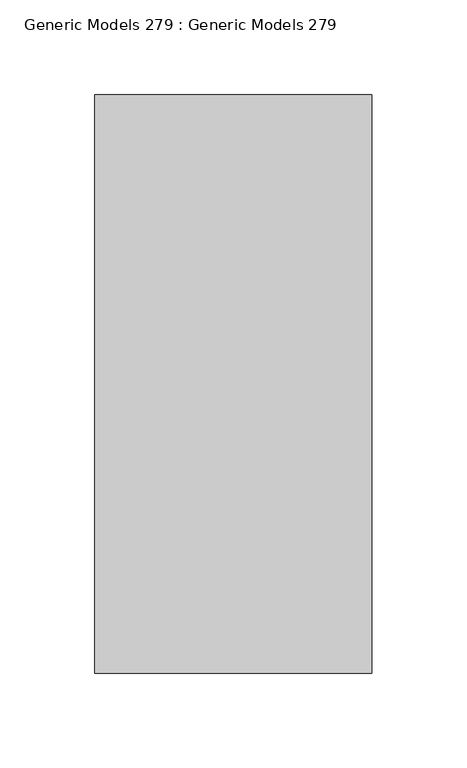
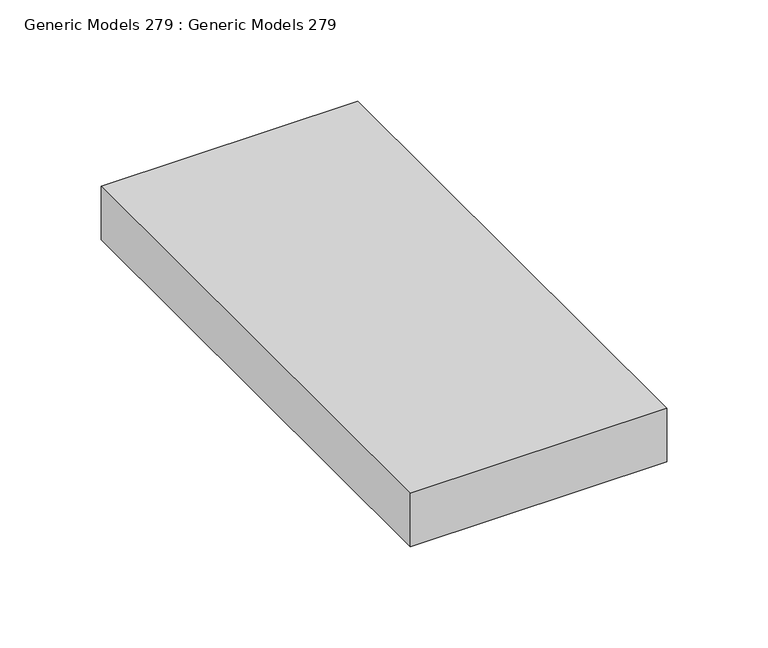
"""IFC4 building model written with IfcOpenShell, lengths in millimetres: proxy geometry, Generic Models 279 : Generic Models 279."""

import ifcopenshell
import ifcopenshell.guid

model = None  # the IFC model being written
_history = None  # IfcOwnerHistory: only IFC2X3 demands one
_inside = {}  # id of a spatial element -> (the spatial element, [elements in it])
_under = {}  # id of a project, library or spatial element -> (it, [spatial elements below it])
_declared = {}  # id of a project -> (the project, [libraries it declares])
_typed = {}  # id of a type object -> (the type object, [elements of that type])
_made_of = {}  # id of a material, layer set ... -> (it, [elements and type objects made of it])


def new_model(schema):
    """Start an empty IFC model of exactly this schema.

    Asked for "IFC4X3", IfcOpenShell would pick the latest addendum, in which some entities
    have other attributes; the version numbers below select the first issue.
    IFC2X3 requires an IfcOwnerHistory on every rooted entity: one is made here for all.
    """
    global model, _history
    if schema == "IFC4X3":
        model = ifcopenshell.file(schema_version=(4, 3, 0, 0))
    else:
        model = ifcopenshell.file(schema=schema)
    _inside.clear()
    _under.clear()
    _declared.clear()
    _typed.clear()
    _made_of.clear()
    _history = None
    if model.schema == "IFC2X3":
        org = make("IfcOrganization", Name="unknown")
        user = make(
            "IfcPersonAndOrganization",
            ThePerson=make("IfcPerson", FamilyName="unknown"),
            TheOrganization=org,
        )
        app = make(
            "IfcApplication",
            ApplicationDeveloper=org,
            Version="unknown",
            ApplicationFullName="unknown",
            ApplicationIdentifier="unknown",
        )
        _history = make(
            "IfcOwnerHistory",
            OwningUser=user,
            OwningApplication=app,
            ChangeAction="ADDED",
            CreationDate=0,
        )
    return model


def make(cls, **values):
    """One entity of the class cls with the attributes given. An attribute that is None is left unset."""
    return model.create_entity(
        cls, **{name: value for name, value in values.items() if value is not None}
    )


def rooted(cls, **values):
    """An entity with a GlobalId (a new one), such as an element, a storey or a relation."""
    return make(cls, GlobalId=ifcopenshell.guid.new(), OwnerHistory=_history, **values)


def si_unit(unit_type, name, prefix=None):
    """IfcSIUnit, for example si_unit("LENGTHUNIT", "METRE", prefix="MILLI")."""
    return make("IfcSIUnit", UnitType=unit_type, Prefix=prefix, Name=name)


def assignment(units):
    """IfcUnitAssignment: the units of a project."""
    return None if units is None else make("IfcUnitAssignment", Units=units)


def point(xyz):
    """IfcCartesianPoint."""
    return None if xyz is None else make("IfcCartesianPoint", Coordinates=xyz)


def direction(xyz):
    """IfcDirection."""
    return None if xyz is None else make("IfcDirection", DirectionRatios=xyz)


def frame(location, z_axis=None, x_axis=None):
    """IfcAxis2Placement3D, a coordinate frame: its origin and axes. An axis left out is left unset."""
    return make(
        "IfcAxis2Placement3D",
        Location=point(location),
        Axis=direction(z_axis),
        RefDirection=direction(x_axis),
    )


def origin():
    """The frame at (0, 0, 0) with its axes left unset."""
    return frame((0.0, 0.0, 0.0))


def place(relative_to, where):
    """IfcLocalPlacement: puts the frame where relative to a parent placement (None: the world)."""
    return make(
        "IfcLocalPlacement", PlacementRelTo=relative_to, RelativePlacement=where
    )


def context(
    kind, dimensions, precision=None, world=None, true_north=None, identifier=None
):
    """IfcGeometricRepresentationContext, for example the 3D "Model" context."""
    return make(
        "IfcGeometricRepresentationContext",
        ContextIdentifier=identifier,
        ContextType=kind,
        CoordinateSpaceDimension=dimensions,
        Precision=precision,
        WorldCoordinateSystem=world,
        TrueNorth=true_north,
    )


def project(units=None, contexts=None):
    """IfcProject with its units and contexts."""
    return rooted(
        "IfcProject",
        Name="project",
        RepresentationContexts=contexts,
        UnitsInContext=assignment(units),
    )


def spatial(cls, under=None, at=None, **own):
    """A site, building, storey or space (cls), placed at a placement, below another one or the project."""
    s = rooted(cls, ObjectPlacement=at, **own)
    if under is not None:
        _under.setdefault(under.id(), (under, []))[1].append(s)
    return s


def polyline(points):
    """IfcPolyline through the points."""
    return make("IfcPolyline", Points=[point(p) for p in points])


def outline(outer, holes=None, kind="AREA"):
    """IfcArbitraryClosedProfileDef: a profile drawn as a closed curve; with holes, ...WithVoids."""
    if holes is None:
        return make("IfcArbitraryClosedProfileDef", ProfileType=kind, OuterCurve=outer)
    return make(
        "IfcArbitraryProfileDefWithVoids",
        ProfileType=kind,
        OuterCurve=outer,
        InnerCurves=holes,
    )


def extrude(swept, where, along, depth):
    """IfcExtrudedAreaSolid: the profile swept, set in the frame where, extruded along a direction by depth."""
    return make(
        "IfcExtrudedAreaSolid",
        SweptArea=swept,
        Position=where,
        ExtrudedDirection=direction(along),
        Depth=depth,
    )


def shape(context_of_items, identifier, shape_type, items):
    """IfcShapeRepresentation: the items that make up one representation, for example the "Body"."""
    return make(
        "IfcShapeRepresentation",
        ContextOfItems=context_of_items,
        RepresentationIdentifier=identifier,
        RepresentationType=shape_type,
        Items=items,
    )


def source(mapping_origin, context_of_items, identifier, shape_type, items):
    """IfcRepresentationMap: a shape defined once, which mapped items show again and again."""
    return make(
        "IfcRepresentationMap",
        MappingOrigin=mapping_origin,
        MappedRepresentation=shape(context_of_items, identifier, shape_type, items),
    )


def transform(
    local_origin,
    x_axis=None,
    y_axis=None,
    z_axis=None,
    scale=None,
    scale2=None,
    scale3=None,
    uniform=True,
):
    """IfcCartesianTransformationOperator3D, or its non-uniform kind. x_axis, y_axis, z_axis: its Axis1, 2, 3."""
    if uniform:
        return make(
            "IfcCartesianTransformationOperator3D",
            Axis1=direction(x_axis),
            Axis2=direction(y_axis),
            LocalOrigin=point(local_origin),
            Scale=scale,
            Axis3=direction(z_axis),
        )
    return make(
        "IfcCartesianTransformationOperator3DnonUniform",
        Axis1=direction(x_axis),
        Axis2=direction(y_axis),
        LocalOrigin=point(local_origin),
        Scale=scale,
        Axis3=direction(z_axis),
        Scale2=scale2,
        Scale3=scale3,
    )


def mapped(mapping_source, mapping_target):
    """IfcMappedItem: shows the shape of a source again, moved by a transform."""
    return make(
        "IfcMappedItem", MappingSource=mapping_source, MappingTarget=mapping_target
    )


def made_of(thing, what):
    """Note that an element or type object is made of a material, layer set ...; save() writes the relation."""
    if what is not None:
        _made_of.setdefault(what.id(), (what, []))[1].append(thing)
    return thing


def element(
    cls,
    number,
    at=None,
    inside=None,
    cuts=None,
    type_object=None,
    material=None,
    context=None,
    identifier="Body",
    shape_type=None,
    held_by="IfcProductDefinitionShape",
    body=None,
    shapes=None,
    **own,
):
    """One element of the class cls, such as IfcWall. Its Tag is "e" and its number.

    at: its placement. inside: the storey or other place that contains it. cuts: it is an
    opening in that element (IfcRelVoidsElement). A single representation is given by context,
    identifier, shape_type and body (its items); several are given by shapes. held_by: the class
    of the entity that holds the representations. save() writes the other relations.
    """
    e = rooted(cls, Tag="e%d" % number, ObjectPlacement=at, **own)
    if body is not None:
        shapes = [shape(context, identifier, shape_type, body)]
    if shapes is not None:
        e.Representation = make(held_by, Representations=shapes)
    if inside is not None:
        _inside.setdefault(inside.id(), (inside, []))[1].append(e)
    if cuts is not None:
        rooted(
            "IfcRelVoidsElement", RelatingBuildingElement=cuts, RelatedOpeningElement=e
        )
    if type_object is not None:
        _typed.setdefault(type_object.id(), (type_object, []))[1].append(e)
    return made_of(e, material)


def aggregate(whole, parts):
    """IfcRelAggregates: a whole, such as a stair, and the parts it consists of."""
    return rooted("IfcRelAggregates", RelatingObject=whole, RelatedObjects=parts)


def save(model, path):
    """Write the relations noted so far, then the file.

    IfcRelAggregates (storeys below a building ...), IfcRelContainedInSpatialStructure (elements
    in a storey), IfcRelDefinesByType, IfcRelAssociatesMaterial and IfcRelDeclares: one each for
    every whole, place, type object, material and project.
    """
    for whole, parts in _under.values():
        aggregate(whole, parts)
    for where, things in _inside.values():
        rooted(
            "IfcRelContainedInSpatialStructure",
            RelatedElements=things,
            RelatingStructure=where,
        )
    for kind, things in _typed.values():
        rooted("IfcRelDefinesByType", RelatedObjects=things, RelatingType=kind)
    for what, things in _made_of.values():
        rooted("IfcRelAssociatesMaterial", RelatedObjects=things, RelatingMaterial=what)
    for by, libraries in _declared.values():
        rooted("IfcRelDeclares", RelatingContext=by, RelatedDefinitions=libraries)
    model.write(path)


def generic_models_279_generic_models_279_9df74be8(model_context):
    return source(origin(), model_context, "Body", "SweptSolid", [
        extrude(outline(polyline([(3531.1804357, 704.5309662), (3677.2304357, 704.5309662), (3677.2304357, 399.7309662), (3531.1804357, 399.7309662), (3531.1804357, 704.5309662)])), frame((0.0, 0.0, 124745.2775398), z_axis=(0.0, 0.0, 1.0), x_axis=(1.0, 0.0, 0.0)), (0.0, 0.0, 1.0), 32.1869688),
    ])


if __name__ == "__main__":
    model = new_model("IFC4")
    model_context = context("Model", 3, world=origin())
    ifc_project = project(units=[si_unit("LENGTHUNIT", "METRE", prefix="MILLI")], contexts=[model_context])
    site = spatial("IfcSite", under=ifc_project)
    building = spatial("IfcBuilding", under=site)
    placement = place(None, origin())
    generic_models_279_generic_models_279_shape = generic_models_279_generic_models_279_9df74be8(model_context)
    element("IfcBuildingElementProxy", 1, Name="Generic Models 279 : Generic Models 279", ObjectType="Generic Models 279 : Generic Models 279", at=placement, inside=building, context=model_context, shape_type="MappedRepresentation", body=[
        mapped(generic_models_279_generic_models_279_shape, transform((0.0, 0.0, 0.0), x_axis=(1.0, 0.0, 0.0), y_axis=(0.0, 1.0, 0.0), z_axis=(0.0, 0.0, 1.0))),
    ])
    save(model, "model.ifc")

# Revit data of these elements
# Element 1 (IfcBuildingElementProxy, "Generic Models 279 : Generic Models 279")
#   Materials on its faces: "_BLOCKING AS REQUIRED"
# Materials
#   "_BLOCKING AS REQUIRED": class "Generic", colour RGB 177 130 114, transparency 0, Cost = 0
